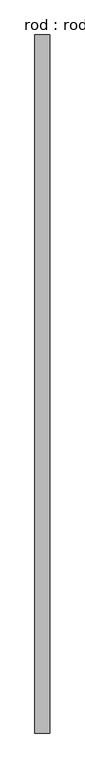
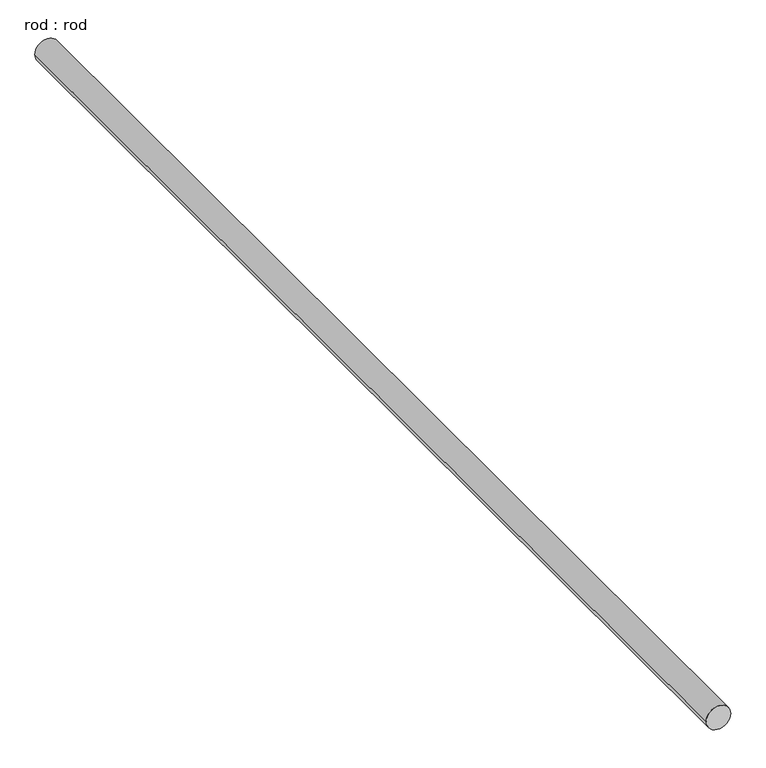
"""IFC4 building model written with IfcOpenShell, lengths in millimetres: proxy geometry, rod : rod."""

import ifcopenshell
import ifcopenshell.guid

model = None  # the IFC model being written
_history = None  # IfcOwnerHistory: only IFC2X3 demands one
_inside = {}  # id of a spatial element -> (the spatial element, [elements in it])
_under = {}  # id of a project, library or spatial element -> (it, [spatial elements below it])
_declared = {}  # id of a project -> (the project, [libraries it declares])
_typed = {}  # id of a type object -> (the type object, [elements of that type])
_made_of = {}  # id of a material, layer set ... -> (it, [elements and type objects made of it])


def new_model(schema):
    """Start an empty IFC model of exactly this schema.

    Asked for "IFC4X3", IfcOpenShell would pick the latest addendum, in which some entities
    have other attributes; the version numbers below select the first issue.
    IFC2X3 requires an IfcOwnerHistory on every rooted entity: one is made here for all.
    """
    global model, _history
    if schema == "IFC4X3":
        model = ifcopenshell.file(schema_version=(4, 3, 0, 0))
    else:
        model = ifcopenshell.file(schema=schema)
    _inside.clear()
    _under.clear()
    _declared.clear()
    _typed.clear()
    _made_of.clear()
    _history = None
    if model.schema == "IFC2X3":
        org = make("IfcOrganization", Name="unknown")
        user = make(
            "IfcPersonAndOrganization",
            ThePerson=make("IfcPerson", FamilyName="unknown"),
            TheOrganization=org,
        )
        app = make(
            "IfcApplication",
            ApplicationDeveloper=org,
            Version="unknown",
            ApplicationFullName="unknown",
            ApplicationIdentifier="unknown",
        )
        _history = make(
            "IfcOwnerHistory",
            OwningUser=user,
            OwningApplication=app,
            ChangeAction="ADDED",
            CreationDate=0,
        )
    return model


def make(cls, **values):
    """One entity of the class cls with the attributes given. An attribute that is None is left unset."""
    return model.create_entity(
        cls, **{name: value for name, value in values.items() if value is not None}
    )


def rooted(cls, **values):
    """An entity with a GlobalId (a new one), such as an element, a storey or a relation."""
    return make(cls, GlobalId=ifcopenshell.guid.new(), OwnerHistory=_history, **values)


def si_unit(unit_type, name, prefix=None):
    """IfcSIUnit, for example si_unit("LENGTHUNIT", "METRE", prefix="MILLI")."""
    return make("IfcSIUnit", UnitType=unit_type, Prefix=prefix, Name=name)


def assignment(units):
    """IfcUnitAssignment: the units of a project."""
    return None if units is None else make("IfcUnitAssignment", Units=units)


def point(xyz):
    """IfcCartesianPoint."""
    return None if xyz is None else make("IfcCartesianPoint", Coordinates=xyz)


def direction(xyz):
    """IfcDirection."""
    return None if xyz is None else make("IfcDirection", DirectionRatios=xyz)


def frame(location, z_axis=None, x_axis=None):
    """IfcAxis2Placement3D, a coordinate frame: its origin and axes. An axis left out is left unset."""
    return make(
        "IfcAxis2Placement3D",
        Location=point(location),
        Axis=direction(z_axis),
        RefDirection=direction(x_axis),
    )


def frame_2d(location, x_axis=None):
    """IfcAxis2Placement2D, a coordinate frame in the plane: its origin and x axis."""
    return make(
        "IfcAxis2Placement2D", Location=point(location), RefDirection=direction(x_axis)
    )


def origin():
    """The frame at (0, 0, 0) with its axes left unset."""
    return frame((0.0, 0.0, 0.0))


def place(relative_to, where):
    """IfcLocalPlacement: puts the frame where relative to a parent placement (None: the world)."""
    return make(
        "IfcLocalPlacement", PlacementRelTo=relative_to, RelativePlacement=where
    )


def context(
    kind, dimensions, precision=None, world=None, true_north=None, identifier=None
):
    """IfcGeometricRepresentationContext, for example the 3D "Model" context."""
    return make(
        "IfcGeometricRepresentationContext",
        ContextIdentifier=identifier,
        ContextType=kind,
        CoordinateSpaceDimension=dimensions,
        Precision=precision,
        WorldCoordinateSystem=world,
        TrueNorth=true_north,
    )


def project(units=None, contexts=None):
    """IfcProject with its units and contexts."""
    return rooted(
        "IfcProject",
        Name="project",
        RepresentationContexts=contexts,
        UnitsInContext=assignment(units),
    )


def spatial(cls, under=None, at=None, **own):
    """A site, building, storey or space (cls), placed at a placement, below another one or the project."""
    s = rooted(cls, ObjectPlacement=at, **own)
    if under is not None:
        _under.setdefault(under.id(), (under, []))[1].append(s)
    return s


def circle_curve(where, radius):
    """IfcCircle in the frame where."""
    return make("IfcCircle", Position=where, Radius=radius)


def trimmed(basis, trim1, trim2, sense, master):
    """IfcTrimmedCurve: the piece of a basis curve between two trims."""
    return make(
        "IfcTrimmedCurve",
        BasisCurve=basis,
        Trim1=trim1,
        Trim2=trim2,
        SenseAgreement=sense,
        MasterRepresentation=master,
    )


def segment(curve, same_sense, transition):
    """IfcCompositeCurveSegment."""
    return make(
        "IfcCompositeCurveSegment",
        Transition=transition,
        SameSense=same_sense,
        ParentCurve=curve,
    )


def composite_curve(segments, self_intersect=None):
    """IfcCompositeCurve: segments joined end to end."""
    return make("IfcCompositeCurve", Segments=segments, SelfIntersect=self_intersect)


def outline(outer, holes=None, kind="AREA"):
    """IfcArbitraryClosedProfileDef: a profile drawn as a closed curve; with holes, ...WithVoids."""
    if holes is None:
        return make("IfcArbitraryClosedProfileDef", ProfileType=kind, OuterCurve=outer)
    return make(
        "IfcArbitraryProfileDefWithVoids",
        ProfileType=kind,
        OuterCurve=outer,
        InnerCurves=holes,
    )


def extrude(swept, where, along, depth):
    """IfcExtrudedAreaSolid: the profile swept, set in the frame where, extruded along a direction by depth."""
    return make(
        "IfcExtrudedAreaSolid",
        SweptArea=swept,
        Position=where,
        ExtrudedDirection=direction(along),
        Depth=depth,
    )


def shape(context_of_items, identifier, shape_type, items):
    """IfcShapeRepresentation: the items that make up one representation, for example the "Body"."""
    return make(
        "IfcShapeRepresentation",
        ContextOfItems=context_of_items,
        RepresentationIdentifier=identifier,
        RepresentationType=shape_type,
        Items=items,
    )


def source(mapping_origin, context_of_items, identifier, shape_type, items):
    """IfcRepresentationMap: a shape defined once, which mapped items show again and again."""
    return make(
        "IfcRepresentationMap",
        MappingOrigin=mapping_origin,
        MappedRepresentation=shape(context_of_items, identifier, shape_type, items),
    )


def transform(
    local_origin,
    x_axis=None,
    y_axis=None,
    z_axis=None,
    scale=None,
    scale2=None,
    scale3=None,
    uniform=True,
):
    """IfcCartesianTransformationOperator3D, or its non-uniform kind. x_axis, y_axis, z_axis: its Axis1, 2, 3."""
    if uniform:
        return make(
            "IfcCartesianTransformationOperator3D",
            Axis1=direction(x_axis),
            Axis2=direction(y_axis),
            LocalOrigin=point(local_origin),
            Scale=scale,
            Axis3=direction(z_axis),
        )
    return make(
        "IfcCartesianTransformationOperator3DnonUniform",
        Axis1=direction(x_axis),
        Axis2=direction(y_axis),
        LocalOrigin=point(local_origin),
        Scale=scale,
        Axis3=direction(z_axis),
        Scale2=scale2,
        Scale3=scale3,
    )


def mapped(mapping_source, mapping_target):
    """IfcMappedItem: shows the shape of a source again, moved by a transform."""
    return make(
        "IfcMappedItem", MappingSource=mapping_source, MappingTarget=mapping_target
    )


def made_of(thing, what):
    """Note that an element or type object is made of a material, layer set ...; save() writes the relation."""
    if what is not None:
        _made_of.setdefault(what.id(), (what, []))[1].append(thing)
    return thing


def element(
    cls,
    number,
    at=None,
    inside=None,
    cuts=None,
    type_object=None,
    material=None,
    context=None,
    identifier="Body",
    shape_type=None,
    held_by="IfcProductDefinitionShape",
    body=None,
    shapes=None,
    **own,
):
    """One element of the class cls, such as IfcWall. Its Tag is "e" and its number.

    at: its placement. inside: the storey or other place that contains it. cuts: it is an
    opening in that element (IfcRelVoidsElement). A single representation is given by context,
    identifier, shape_type and body (its items); several are given by shapes. held_by: the class
    of the entity that holds the representations. save() writes the other relations.
    """
    e = rooted(cls, Tag="e%d" % number, ObjectPlacement=at, **own)
    if body is not None:
        shapes = [shape(context, identifier, shape_type, body)]
    if shapes is not None:
        e.Representation = make(held_by, Representations=shapes)
    if inside is not None:
        _inside.setdefault(inside.id(), (inside, []))[1].append(e)
    if cuts is not None:
        rooted(
            "IfcRelVoidsElement", RelatingBuildingElement=cuts, RelatedOpeningElement=e
        )
    if type_object is not None:
        _typed.setdefault(type_object.id(), (type_object, []))[1].append(e)
    return made_of(e, material)


def aggregate(whole, parts):
    """IfcRelAggregates: a whole, such as a stair, and the parts it consists of."""
    return rooted("IfcRelAggregates", RelatingObject=whole, RelatedObjects=parts)


def save(model, path):
    """Write the relations noted so far, then the file.

    IfcRelAggregates (storeys below a building ...), IfcRelContainedInSpatialStructure (elements
    in a storey), IfcRelDefinesByType, IfcRelAssociatesMaterial and IfcRelDeclares: one each for
    every whole, place, type object, material and project.
    """
    for whole, parts in _under.values():
        aggregate(whole, parts)
    for where, things in _inside.values():
        rooted(
            "IfcRelContainedInSpatialStructure",
            RelatedElements=things,
            RelatingStructure=where,
        )
    for kind, things in _typed.values():
        rooted("IfcRelDefinesByType", RelatedObjects=things, RelatingType=kind)
    for what, things in _made_of.values():
        rooted("IfcRelAssociatesMaterial", RelatedObjects=things, RelatingMaterial=what)
    for by, libraries in _declared.values():
        rooted("IfcRelDeclares", RelatingContext=by, RelatedDefinitions=libraries)
    model.write(path)


def rod_rod_cd846f51(model_context):
    return source(origin(), model_context, "Body", "SweptSolid", [
        extrude(outline(composite_curve([segment(trimmed(circle_curve(frame_2d((0.0108462, 0.0)), 200.0), [point((0.0108462, 200.0))], [point((0.0108462, -200.0))], False, "CARTESIAN"), True, "CONTINUOUS"), segment(trimmed(circle_curve(frame_2d((0.0108462, 0.0)), 200.0), [point((0.0108462, -200.0))], [point((0.0108462, 200.0))], False, "CARTESIAN"), True, "CONTINUOUS")], self_intersect=False)), frame((0.0, -5402.8070989, 0.0), z_axis=(0.0, 1.0, 0.0), x_axis=(0.0, 0.0, 1.0)), (0.0, 0.0, 1.0), 18991.0714286),
    ])


if __name__ == "__main__":
    model = new_model("IFC4")
    model_context = context("Model", 3, world=origin())
    ifc_project = project(units=[si_unit("LENGTHUNIT", "METRE", prefix="MILLI")], contexts=[model_context])
    site = spatial("IfcSite", under=ifc_project)
    building = spatial("IfcBuilding", under=site)
    placement = place(None, origin())
    rod_rod_shape = rod_rod_cd846f51(model_context)
    element("IfcBuildingElementProxy", 1, Name="rod : rod", ObjectType="rod : rod", at=placement, inside=building, context=model_context, shape_type="MappedRepresentation", body=[
        mapped(rod_rod_shape, transform((0.0, 0.0, 0.0), x_axis=(1.0, 0.0, 0.0), y_axis=(0.0, 1.0, 0.0), z_axis=(0.0, 0.0, 1.0))),
    ])
    save(model, "model.ifc")

# Revit data of these elements
# Type "rod : rod"
#   Default Elevation = 0
